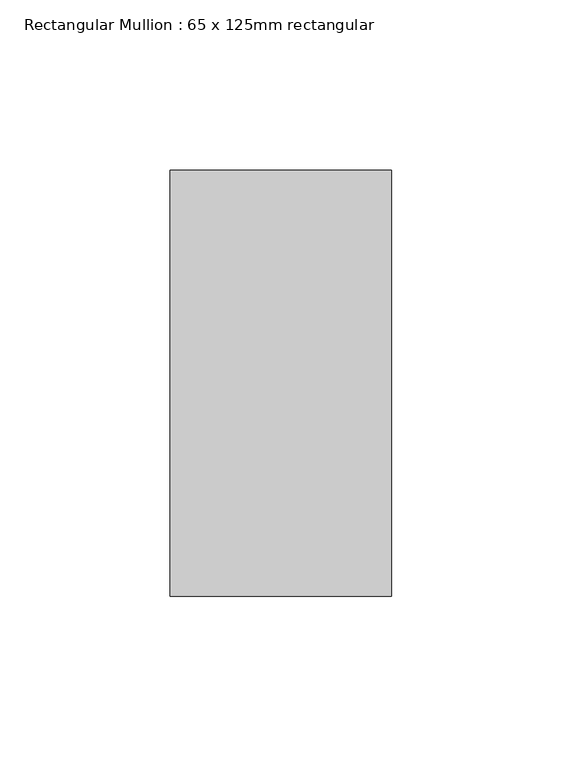
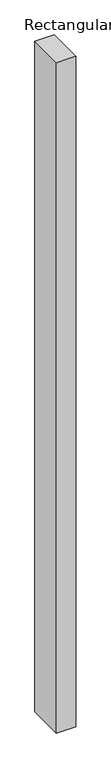
"""IFC4 building model written with IfcOpenShell, lengths in millimetres: member geometry, Rectangular Mullion : 65 x 125mm rectangular."""

from ifc_helpers import new_model, si_unit, frame, origin, place, context, project, spatial, polyline, outline, extrude, source, transform, mapped, element, save


def rectangular_mullion_65_x_125mm_rectangular_944d97ce(model_context):
    return source(origin(), model_context, "Body", "SweptSolid", [
        extrude(outline(polyline([(0.0, 62.5), (0.0, -62.5), (-65.0, -62.5), (-65.0, 62.5), (0.0, 62.5)])), frame((0.0, 0.0, -2373.0683182), z_axis=(0.0, 0.0, 1.0), x_axis=(1.0, 0.0, 0.0)), (0.0, 0.0, 1.0), 2373.0683182),
    ])


if __name__ == "__main__":
    model = new_model("IFC4")
    model_context = context("Model", 3, world=origin())
    ifc_project = project(units=[si_unit("LENGTHUNIT", "METRE", prefix="MILLI")], contexts=[model_context])
    site = spatial("IfcSite", under=ifc_project)
    building = spatial("IfcBuilding", under=site)
    placement = place(None, origin())
    rectangular_mullion_65_x_125mm_rectangular_shape = rectangular_mullion_65_x_125mm_rectangular_944d97ce(model_context)
    element("IfcMember", 1, ObjectType="Rectangular Mullion : 65 x 125mm rectangular", at=placement, inside=building, context=model_context, shape_type="MappedRepresentation", body=[
        mapped(rectangular_mullion_65_x_125mm_rectangular_shape, transform((0.0, 0.0, 0.0), x_axis=(1.0, 0.0, 0.0), y_axis=(0.0, 1.0, 0.0), z_axis=(0.0, 0.0, 1.0))),
    ])
    save(model, "model.ifc")

# Revit data of these elements
# Type "Rectangular Mullion : 65 x 125mm rectangular"
#   built-in parameter 1007304 = 0.410105 (stored number, unit not read)
#   built-in parameter 1007301 = 0.106627 (stored number, unit not read)
#   built-in parameter 1007300 = 0.106627 (stored number, unit not read)
# Element 1 (IfcMember, "Rectangular Mullion : 65 x 125mm rectangular")
#   Materials on its faces: "Aluminum"
# Materials
#   "Aluminum": class "Metal", colour RGB 244 245 246, transparency 0, Description = "Aluminum 6061", Cost = 0
